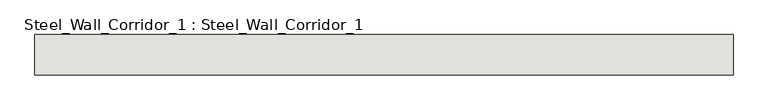
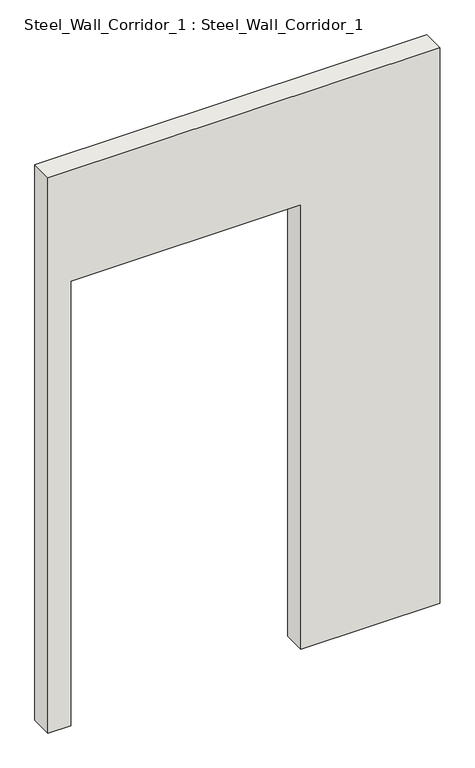
"""IFC4 building model written with IfcOpenShell, lengths in millimetres: wall geometry, Steel_Wall_Corridor_1 : Steel_Wall_Corridor_1."""

from ifc_helpers import new_model, si_unit, frame, origin, place, context, project, spatial, polyline, outline, extrude, source, transform, mapped, element, save


def steel_wall_corridor_1_steel_wall_corridor_1_64942479(model_context):
    return source(origin(), model_context, "Body", "SweptSolid", [
        extrude(outline(polyline([(2850.0, 1950.0), (2850.0, 215.0), (250.0, 215.0), (250.0, 315.0), (2330.0, 315.0), (2330.0, 1335.0), (250.0, 1335.0), (250.0, 1950.0), (2850.0, 1950.0)])), frame((0.0, 3475.0, 0.0), z_axis=(0.0, 1.0, 0.0), x_axis=(0.0, 0.0, 1.0)), (0.0, 0.0, 1.0), 100.0),
    ])


if __name__ == "__main__":
    model = new_model("IFC4")
    model_context = context("Model", 3, world=origin())
    ifc_project = project(units=[si_unit("LENGTHUNIT", "METRE", prefix="MILLI")], contexts=[model_context])
    site = spatial("IfcSite", under=ifc_project)
    building = spatial("IfcBuilding", under=site)
    placement = place(None, origin())
    steel_wall_corridor_1_steel_wall_corridor_1_shape = steel_wall_corridor_1_steel_wall_corridor_1_64942479(model_context)
    element("IfcWall", 1, ObjectType="Steel_Wall_Corridor_1 : Steel_Wall_Corridor_1", at=placement, inside=building, context=model_context, shape_type="MappedRepresentation", body=[
        mapped(steel_wall_corridor_1_steel_wall_corridor_1_shape, transform((0.0, 0.0, 0.0), x_axis=(1.0, 0.0, 0.0), y_axis=(0.0, 1.0, 0.0), z_axis=(0.0, 0.0, 1.0))),
    ])
    save(model, "model.ifc")

# Revit data of these elements
# Type "Steel_Wall_Corridor_1 : Steel_Wall_Corridor_1"
#   NameOverride = "Steel_Wall_Corridor_1"
# Element 1 (IfcWall, "Steel_Wall_Corridor_1 : Steel_Wall_Corridor_1")
#   Materials on its faces: "IfcSurfaceStyle #33"
# Materials
#   "IfcSurfaceStyle #33": class "Unassigned", colour RGB 214 214 214, transparency 0
